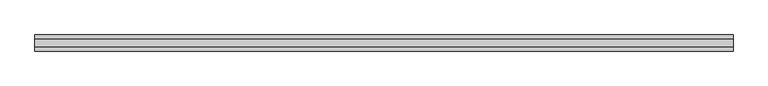
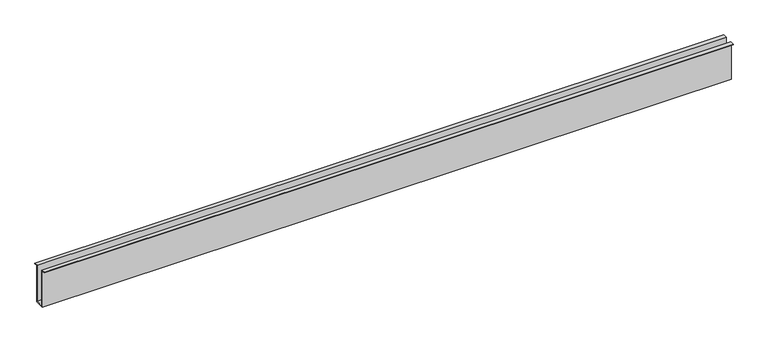
"""IFC4 building model written with IfcOpenShell, lengths in millimetres: railing geometry, ML_Perfil U de embutir1 : ML_Perfil U de embutir."""

from ifc_helpers import new_model, si_unit, frame, origin, place, context, project, spatial, polyline, outline, extrude, source, transform, mapped, element, save


def railing_4d275163(model_context):
    return source(origin(), model_context, "Body", "SweptSolid", [
        extrude(outline(polyline([(1832.4523952, 3702.0), (1832.4523952, 3594.0), (1856.4523952, 3594.0), (1856.4523952, 3702.0), (1866.9523952, 3702.0), (1866.9523952, 3700.0), (1858.4523952, 3700.0), (1858.4523952, 3592.0), (1830.4523952, 3592.0), (1830.4523952, 3700.0), (1821.9523952, 3700.0), (1821.9523952, 3702.0), (1832.4523952, 3702.0)])), frame((-12226.1487231, 0.0, 0.0), z_axis=(1.0, 0.0, 0.0), x_axis=(0.0, 1.0, 0.0)), (0.0, 0.0, 1.0), 1950.0),
    ])


if __name__ == "__main__":
    model = new_model("IFC4")
    model_context = context("Model", 3, world=origin())
    ifc_project = project(units=[si_unit("LENGTHUNIT", "METRE", prefix="MILLI")], contexts=[model_context])
    site = spatial("IfcSite", under=ifc_project)
    building = spatial("IfcBuilding", under=site)
    placement = place(None, origin())
    railing_shape = railing_4d275163(model_context)
    element("IfcRailing", 1, ObjectType="ML_Perfil U de embutir1 : ML_Perfil U de embutir", at=placement, inside=building, context=model_context, shape_type="MappedRepresentation", body=[
        mapped(railing_shape, transform((0.0, 0.0, 0.0), x_axis=(1.0, 0.0, 0.0), y_axis=(0.0, 1.0, 0.0), z_axis=(0.0, 0.0, 1.0))),
    ])
    save(model, "model.ifc")

# Revit data of these elements
# Type "ML_Perfil U de embutir1 : ML_Perfil U de embutir"
#   ME_Compr [instance default] = 1.95 m
#   ME_Material Perfil [instance default] = .ALUMÍNIO COM PINTURA ELETROSTÁTICA BRANCA
# Element 1 (IfcRailing, "ML_Perfil U de embutir1 : ML_Perfil U de embutir")
#   Materials on its faces: ".ALUMÍNIO COM PINTURA ELETROSTÁTICA BRANCA"
# Materials
#   ".ALUMÍNIO COM PINTURA ELETROSTÁTICA BRANCA": class "CC_METAIS", colour RGB 241 241 241, transparency 0, Cost = 0
